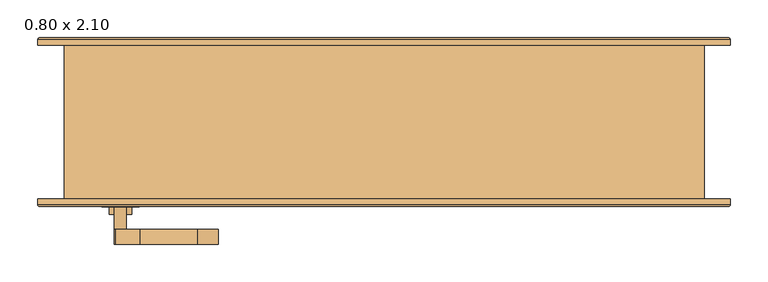
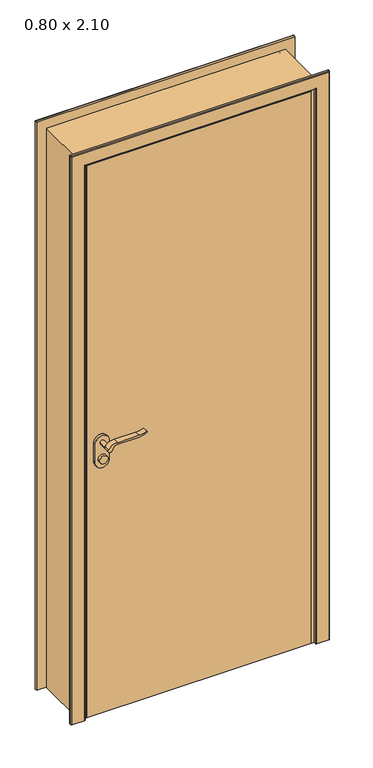
"""IFC4 building model written with IfcOpenShell, lengths in millimetres: door geometry, .CC_ND 300_PORTA SIMPLES DE ABRIR_COM EXTENSÃO : 0.80 x 2.10."""

from ifc_helpers import new_model, si_unit, point, frame, frame_2d, origin, origin_with_axes, place, context, project, spatial, polyline, circle_curve, ellipse_curve, trimmed, segment, composite_curve, outline, extrude, faceted_brep, source, transform, mapped, element, save
from ifc_brep_helpers import plane_surface, cylinder_surface, advanced_brep


def door_0_80_x_2_10_5db6a8b4(model_context):
    return source(origin(), model_context, "Body", "SolidModel", [
        extrude(outline(composite_curve([segment(trimmed(circle_curve(frame_2d((964.5, -350.0)), 15.0), [point((964.5, -335.0))], [point((964.5, -365.0))], False, "CARTESIAN"), True, "CONTINUOUS"), segment(trimmed(circle_curve(frame_2d((964.5, -350.0)), 15.0), [point((964.5, -365.0))], [point((964.5, -335.0))], False, "CARTESIAN"), True, "CONTINUOUS")], self_intersect=False)), frame((0.0, -137.9, 0.0), z_axis=(0.0, 1.0, 0.0), x_axis=(0.0, 0.0, 1.0)), (0.0, 0.0, 1.0), 10.0),
        extrude(outline(composite_curve([segment(trimmed(circle_curve(frame_2d((964.5, -350.0)), 15.0), [point((964.5, -335.0))], [point((964.5, -365.0))], False, "CARTESIAN"), True, "CONTINUOUS"), segment(trimmed(circle_curve(frame_2d((964.5, -350.0)), 15.0), [point((964.5, -365.0))], [point((964.5, -335.0))], False, "CARTESIAN"), True, "CONTINUOUS")], self_intersect=False)), frame((0.0, -77.9, 0.0), z_axis=(0.0, 1.0, 0.0), x_axis=(0.0, 0.0, 1.0)), (0.0, 0.0, 1.0), 10.0),
        extrude(outline(composite_curve([segment(trimmed(circle_curve(frame_2d((1024.5, -350.0)), 8.0), [point((1029.1523287, -356.5081363))], [point((1024.5, -342.0))], False, "CARTESIAN"), True, "CONTINUOUS"), segment(trimmed(circle_curve(frame_2d((1019.3738613, -324.6138099)), 18.1261387), [point((1024.5, -342.0))], [point((1037.5, -324.6138099))], True, "CARTESIAN"), True, "CONTINUOUS"), segment(polyline([(1037.5, -324.6138099), (1037.5, -248.3564091)]), True, "CONTINUOUS"), segment(trimmed(circle_curve(frame_2d((1096.7709207, -251.9396612)), 59.3791355), [point((1037.5, -248.3564091))], [point((1046.7135558, -220.0))], False, "CARTESIAN"), True, "CONTINUOUS"), segment(polyline([(1046.7135558, -220.0), (1049.5, -220.0)]), True, "CONTINUOUS"), segment(trimmed(circle_curve(frame_2d((1127.7850638, -248.4227909)), 83.2850902), [point((1049.5, -220.0))], [point((1044.5, -248.3564091))], True, "CARTESIAN"), True, "CONTINUOUS"), segment(polyline([(1044.5, -248.3564091), (1044.5, -324.6325667)]), True, "CONTINUOUS"), segment(trimmed(circle_curve(frame_2d((1007.2555521, -326.3324871)), 37.2832219), [point((1044.5, -324.6325667))], [point((1029.1523287, -356.5081363))], False, "CARTESIAN"), True, "CONTINUOUS")], self_intersect=False)), frame((0.0, -177.9, 0.0), z_axis=(0.0, 1.0, 0.0), x_axis=(0.0, 0.0, 1.0)), (0.0, 0.0, 1.0), 20.0),
        extrude(outline(composite_curve([segment(trimmed(circle_curve(frame_2d((1019.3738682, -324.6138122)), 18.1261318), [point((1024.4999903, -342.0))], [point((1037.5, -324.6138122))], True, "CARTESIAN"), True, "CONTINUOUS"), segment(polyline([(1037.5, -324.6138122), (1037.5, -248.3564091)]), True, "CONTINUOUS"), segment(trimmed(circle_curve(frame_2d((1096.7709207, -251.9396612)), 59.3791355), [point((1037.5, -248.3564091))], [point((1046.7135558, -220.0))], False, "CARTESIAN"), True, "CONTINUOUS"), segment(polyline([(1046.7135558, -220.0), (1049.5, -220.0)]), True, "CONTINUOUS"), segment(trimmed(circle_curve(frame_2d((1127.7850638, -248.4227909)), 83.2850902), [point((1049.5, -220.0))], [point((1044.5, -248.3564091))], True, "CARTESIAN"), True, "CONTINUOUS"), segment(polyline([(1044.5, -248.3564091), (1044.5, -324.6325667)]), True, "CONTINUOUS"), segment(trimmed(circle_curve(frame_2d((1007.2555521, -326.3324871)), 37.2832219), [point((1044.5, -324.6325667))], [point((1029.1523287, -356.5081363))], False, "CARTESIAN"), True, "CONTINUOUS"), segment(trimmed(circle_curve(frame_2d((1024.5, -350.0)), 8.0), [point((1029.1523287, -356.5081363))], [point((1024.4999903, -342.0))], False, "CARTESIAN"), True, "CONTINUOUS")], self_intersect=False)), frame((0.0, -47.9, 0.0), z_axis=(0.0, 1.0, 0.0), x_axis=(0.0, 0.0, 1.0)), (0.0, 0.0, 1.0), 20.0),
        extrude(outline(composite_curve([segment(trimmed(circle_curve(frame_2d((1024.5, -350.0)), 8.0), [point((1024.5, -342.0))], [point((1024.5, -358.0))], False, "CARTESIAN"), True, "CONTINUOUS"), segment(trimmed(circle_curve(frame_2d((1024.5, -350.0)), 8.0), [point((1024.5, -358.0))], [point((1024.5, -342.0))], False, "CARTESIAN"), True, "CONTINUOUS")], self_intersect=False)), frame((0.0, -157.9, 0.0), z_axis=(0.0, 1.0, 0.0), x_axis=(0.0, 0.0, 1.0)), (0.0, 0.0, 1.0), 30.0),
        extrude(outline(composite_curve([segment(trimmed(circle_curve(frame_2d((1024.5, -350.0)), 8.0), [point((1024.5, -342.0))], [point((1024.5, -358.0))], False, "CARTESIAN"), True, "CONTINUOUS"), segment(trimmed(circle_curve(frame_2d((1024.5, -350.0)), 8.0), [point((1024.5, -358.0))], [point((1024.5, -342.0))], False, "CARTESIAN"), True, "CONTINUOUS")], self_intersect=False)), frame((0.0, -77.9, 0.0), z_axis=(0.0, 1.0, 0.0), x_axis=(0.0, 0.0, 1.0)), (0.0, 0.0, 1.0), 30.0),
        extrude(outline(composite_curve([segment(trimmed(circle_curve(frame_2d((954.5, -350.0)), 25.0), [point((954.5, -375.0))], [point((954.5, -325.0))], False, "CARTESIAN"), True, "CONTINUOUS"), segment(polyline([(954.5, -325.0), (1024.5, -325.0)]), True, "CONTINUOUS"), segment(trimmed(circle_curve(frame_2d((1024.5, -350.0)), 25.0), [point((1024.5, -325.0))], [point((1024.5, -375.0))], False, "CARTESIAN"), True, "CONTINUOUS"), segment(polyline([(1024.5, -375.0), (954.5, -375.0)]), True, "CONTINUOUS")], self_intersect=False)), frame((0.0, -127.9, 0.0), z_axis=(0.0, 1.0, 0.0), x_axis=(0.0, 0.0, 1.0)), (0.0, 0.0, 1.0), 10.0),
        extrude(outline(composite_curve([segment(trimmed(circle_curve(frame_2d((954.5, -350.0)), 25.0), [point((954.5, -375.0))], [point((954.5, -325.0))], False, "CARTESIAN"), True, "CONTINUOUS"), segment(polyline([(954.5, -325.0), (1024.5, -325.0)]), True, "CONTINUOUS"), segment(trimmed(circle_curve(frame_2d((1024.5, -350.0)), 25.0), [point((1024.5, -325.0))], [point((1024.5, -375.0))], False, "CARTESIAN"), True, "CONTINUOUS"), segment(polyline([(1024.5, -375.0), (954.5, -375.0)]), True, "CONTINUOUS")], self_intersect=False)), frame((0.0, -87.9, 0.0), z_axis=(0.0, 1.0, 0.0), x_axis=(0.0, 0.0, 1.0)), (0.0, 0.0, 1.0), 10.0),
        faceted_brep([(392.0, 86.9, 0.0), (425.0, 86.9, 0.0), (425.0, -117.9, 0.0), (400.0, -117.9, 0.0), (400.0, -87.9, 0.0), (392.0, -87.9, 0.0), (392.0, 86.9, 2067.0), (-392.0, 86.9, 2067.0), (-392.0, 86.9, 0.0), (-425.0, 86.9, 0.0), (-425.0, 86.9, 2100.0), (425.0, 86.9, 2100.0), (425.0, -117.9, 2100.0), (-425.0, -117.9, 2100.0), (-425.0, -117.9, 0.0), (-400.0, -117.9, 0.0), (-400.0, -117.9, 2075.0), (400.0, -117.9, 2075.0), (400.0, -87.9, 2075.0), (-400.0, -87.9, 2075.0), (-400.0, -87.9, 0.0), (-392.0, -87.9, 0.0), (-392.0, -87.9, 2067.0), (392.0, -87.9, 2067.0)], [[[0, 1, 2, 3, 4, 5]], [[1, 0, 6, 7, 8, 9, 10, 11]], [[2, 1, 11, 12]], [[3, 2, 12, 13, 14, 15, 16, 17]], [[4, 3, 17, 18]], [[5, 4, 18, 19, 20, 21, 22, 23]], [[0, 5, 23, 6]], [[7, 22, 21, 8]], [[8, 21, 20, 15, 14, 9]], [[13, 10, 9, 14]], [[19, 16, 15, 20]], [[12, 11, 10, 13]], [[18, 17, 16, 19]], [[6, 23, 22, 7]]]),
        extrude(outline(polyline([(-400.0, -87.9), (400.0, -87.9), (400.0, -117.9), (-400.0, -117.9), (-400.0, -87.9)])), origin_with_axes(), (0.0, 0.0, 1.0), 2075.0),
        advanced_brep(
        [(-460.0, -117.9, 0.0), (-410.0, -117.9, 0.0), (-410.0, -124.9, 0.0), (-413.0, -127.9, 0.0), (-457.0, -127.9, 0.0), (-460.0, -124.9, 0.0), (-460.0, -117.9, 2135.0), (460.0, -117.9, 2135.0), (460.0, -117.9, 0.0), (410.0, -117.9, 0.0), (410.0, -117.9, 2085.0), (-410.0, -117.9, 2085.0), (-410.0, -124.9, 2085.0), (-413.0, -127.9, 2088.0), (413.0, -127.9, 2088.0), (413.0, -127.9, 0.0), (457.0, -127.9, 0.0), (457.0, -127.9, 2132.0), (-457.0, -127.9, 2132.0), (-460.0, -124.9, 2135.0), (460.0, -124.9, 2135.0), (460.0, -124.9, 0.0), (410.0, -124.9, 0.0), (410.0, -124.9, 2085.0)],
        [
            (0, 1),
            (1, 2),
            (2, 3, circle_curve(frame((-413.0, -124.9, 0.0), z_axis=(0.0, 0.0, -1.0), x_axis=(1.0, 0.0, 0.0)), 3.0)),
            (3, 4),
            (4, 5, circle_curve(frame((-457.0, -124.9, 0.0), z_axis=(0.0, 0.0, -1.0), x_axis=(1.0, 0.0, 0.0)), 3.0)),
            (5, 0),
            (0, 6),
            (6, 7),
            (7, 8),
            (8, 9),
            (9, 10),
            (10, 11),
            (11, 1),
            (11, 12),
            (12, 2),
            (12, 13, ellipse_curve(frame((-413.0, -124.9, 2088.0), z_axis=(-0.7071067811865475, 0.0, -0.7071067811865475), x_axis=(0.7071067811865474, 0.0, -0.7071067811865476)), 4.2426407, 3.0)),
            (13, 3),
            (13, 14),
            (14, 15),
            (15, 16),
            (16, 17),
            (17, 18),
            (18, 4),
            (18, 19, ellipse_curve(frame((-457.0, -124.9, 2132.0), z_axis=(-0.7071067811865475, 0.0, -0.7071067811865475), x_axis=(0.7071067811865474, 0.0, -0.7071067811865476)), 4.2426407, 3.0)),
            (19, 5),
            (19, 6),
            (7, 20),
            (20, 21),
            (21, 8),
            (21, 16, circle_curve(frame((457.0, -124.9, 0.0), z_axis=(0.0, 0.0, -1.0), x_axis=(-1.0, 0.0, 0.0)), 3.0)),
            (15, 22, circle_curve(frame((413.0, -124.9, 0.0), z_axis=(0.0, 0.0, -1.0), x_axis=(-1.0, 0.0, 0.0)), 3.0)),
            (22, 9),
            (23, 10),
            (22, 23),
            (14, 23, ellipse_curve(frame((413.0, -124.9, 2088.0), z_axis=(0.7071067811865475, 0.0, -0.7071067811865475), x_axis=(0.7071067811865474, 0.0, 0.7071067811865476)), 4.2426407, 3.0)),
            (20, 17, ellipse_curve(frame((457.0, -124.9, 2132.0), z_axis=(0.7071067811865475, 0.0, -0.7071067811865475), x_axis=(0.7071067811865474, 0.0, 0.7071067811865476)), 4.2426407, 3.0)),
            (23, 12),
            (19, 20),
        ],
        [
            plane_surface(frame((-410.0, -117.9, 0.0), z_axis=(0.0, 0.0, -1.0), x_axis=(0.0, 1.0, 0.0))),
            plane_surface(frame((-460.0, -117.9, 0.0), z_axis=(0.0, 1.0, 0.0), x_axis=(0.0, 0.0, 1.0))),
            plane_surface(frame((-410.0, -117.9, 0.0), z_axis=(1.0, 0.0, 0.0), x_axis=(0.0, 0.0, 1.0))),
            cylinder_surface(frame((-413.0, -124.9, 0.0), z_axis=(0.0, 0.0, -1.0), x_axis=(1.0, 0.0, 0.0)), 3.0),
            plane_surface(frame((-413.0, -127.9, 0.0), z_axis=(0.0, -1.0, 0.0), x_axis=(0.0, 0.0, 1.0))),
            cylinder_surface(frame((-457.0, -124.9, 0.0), z_axis=(0.0, 0.0, -1.0), x_axis=(1.0, 0.0, 0.0)), 3.0),
            plane_surface(frame((-460.0, -124.9, 0.0), z_axis=(-1.0, 0.0, 0.0), x_axis=(0.0, 0.0, 1.0))),
            plane_surface(frame((460.0, -124.9, 2135.0), z_axis=(1.0, 0.0, 0.0), x_axis=(0.0, 0.0, -1.0))),
            plane_surface(frame((410.0, -117.9, 0.0), z_axis=(0.0, 0.0, -1.0), x_axis=(0.0, 1.0, 0.0))),
            plane_surface(frame((410.0, -117.9, 2085.0), z_axis=(-1.0, 0.0, 0.0), x_axis=(0.0, 0.0, -1.0))),
            cylinder_surface(frame((413.0, -124.9, 2085.0), z_axis=(0.0, 0.0, 1.0), x_axis=(-1.0, 0.0, 0.0)), 3.0),
            cylinder_surface(frame((457.0, -124.9, 2085.0), z_axis=(0.0, 0.0, 1.0), x_axis=(-1.0, 0.0, 0.0)), 3.0),
            plane_surface(frame((-410.0, -117.9, 2085.0), z_axis=(0.0, 0.0, -1.0), x_axis=(1.0, 0.0, 0.0))),
            plane_surface(frame((-460.0, -124.9, 2135.0), z_axis=(0.0, 0.0, 1.0), x_axis=(1.0, 0.0, 0.0))),
            cylinder_surface(frame((-410.0, -124.9, 2088.0), z_axis=(-1.0, 0.0, 0.0), x_axis=(0.0, 0.0, -1.0)), 3.0),
            cylinder_surface(frame((-410.0, -124.9, 2132.0), z_axis=(-1.0, 0.0, 0.0), x_axis=(0.0, 0.0, -1.0)), 3.0),
        ],
        [
            (0, [[1, 2, 3, 4, 5, 6]]),
            (1, [[-1, 7, 8, 9, 10, 11, 12, 13]]),
            (2, [[-2, -13, 14, 15]]),
            (3, [[-3, -15, 16, 17]]),
            (4, [[-4, -17, 18, 19, 20, 21, 22, 23]]),
            (5, [[-5, -23, 24, 25]]),
            (6, [[-6, -25, 26, -7]]),
            (7, [[27, 28, 29, -9]]),
            (8, [[-29, 30, -20, 31, 32, -10]]),
            (9, [[33, -11, -32, 34]]),
            (10, [[35, -34, -31, -19]]),
            (11, [[36, -21, -30, -28]]),
            (12, [[-14, -12, -33, 37]]),
            (13, [[-26, 38, -27, -8]]),
            (14, [[-16, -37, -35, -18]]),
            (15, [[-24, -22, -36, -38]]),
        ],
    ),
        advanced_brep(
        [(460.0, 86.9, 0.0), (410.0, 86.9, 0.0), (410.0, 93.9157283, 0.0), (412.9842717, 96.9, 0.0), (457.0342217, 96.9, 0.0), (460.0, 93.9342217, 0.0), (460.0, 86.9, 2135.0), (-460.0, 86.9, 2135.0), (-460.0, 86.9, 0.0), (-410.0, 86.9, 0.0), (-410.0, 86.9, 2085.0), (410.0, 86.9, 2085.0), (410.0, 93.9157283, 2085.0), (412.9842717, 96.9, 2087.9842717), (-412.9842717, 96.9, 2087.9842717), (-412.9842717, 96.9, 0.0), (-457.0342217, 96.9, 0.0), (-457.0342217, 96.9, 2132.0342217), (457.0342217, 96.9, 2132.0342217), (460.0, 93.9342217, 2135.0), (-460.0, 93.9342217, 2135.0), (-460.0, 93.9342217, 0.0), (-410.0, 93.9157283, 0.0), (-410.0, 93.9157283, 2085.0)],
        [
            (0, 1),
            (1, 2),
            (2, 3, circle_curve(frame((412.9842717, 93.9157283, 0.0), z_axis=(0.0, 0.0, -1.0), x_axis=(1.0, 0.0, 0.0)), 2.9842717)),
            (3, 4),
            (4, 5, circle_curve(frame((457.0342217, 93.9342217, 0.0), z_axis=(0.0, 0.0, -1.0), x_axis=(1.0, 0.0, 0.0)), 2.9657783)),
            (5, 0),
            (0, 6),
            (6, 7),
            (7, 8),
            (8, 9),
            (9, 10),
            (10, 11),
            (11, 1),
            (11, 12),
            (12, 2),
            (12, 13, ellipse_curve(frame((412.9842717, 93.9157283, 2087.9842717), z_axis=(0.7071067811865475, 0.0, -0.7071067811865475), x_axis=(-0.7071067811865474, 0.0, -0.7071067811865476)), 4.2203975, 2.9842717)),
            (13, 3),
            (13, 14),
            (14, 15),
            (15, 16),
            (16, 17),
            (17, 18),
            (18, 4),
            (18, 19, ellipse_curve(frame((457.0342217, 93.9342217, 2132.0342217), z_axis=(0.7071067811865475, 0.0, -0.7071067811865475), x_axis=(-0.7071067811865474, 0.0, -0.7071067811865476)), 4.1942438, 2.9657783)),
            (19, 5),
            (19, 6),
            (7, 20),
            (20, 21),
            (21, 8),
            (21, 16, circle_curve(frame((-457.0342217, 93.9342217, 0.0), z_axis=(0.0, 0.0, -1.0), x_axis=(-1.0, 0.0, 0.0)), 2.9657783)),
            (15, 22, circle_curve(frame((-412.9842717, 93.9157283, 0.0), z_axis=(0.0, 0.0, -1.0), x_axis=(-1.0, 0.0, 0.0)), 2.9842717)),
            (22, 9),
            (23, 10),
            (22, 23),
            (14, 23, ellipse_curve(frame((-412.9842717, 93.9157283, 2087.9842717), z_axis=(-0.7071067811865475, 0.0, -0.7071067811865475), x_axis=(-0.7071067811865474, 0.0, 0.7071067811865476)), 4.2203975, 2.9842717)),
            (20, 17, ellipse_curve(frame((-457.0342217, 93.9342217, 2132.0342217), z_axis=(-0.7071067811865475, 0.0, -0.7071067811865475), x_axis=(-0.7071067811865474, 0.0, 0.7071067811865476)), 4.1942438, 2.9657783)),
            (23, 12),
            (19, 20),
        ],
        [
            plane_surface(frame((410.0, 86.9, 0.0), z_axis=(0.0, 0.0, -1.0), x_axis=(0.0, 1.0, 0.0))),
            plane_surface(frame((460.0, 86.9, 0.0), z_axis=(0.0, -1.0, 0.0), x_axis=(0.0, 0.0, 1.0))),
            plane_surface(frame((410.0, 86.9, 0.0), z_axis=(-1.0, 0.0, 0.0), x_axis=(0.0, 0.0, 1.0))),
            cylinder_surface(frame((412.9842717, 93.9157283, 0.0), z_axis=(0.0, 0.0, -1.0), x_axis=(1.0, 0.0, 0.0)), 2.9842717),
            plane_surface(frame((412.9842717, 96.9, 0.0), z_axis=(0.0, 1.0, 0.0), x_axis=(0.0, 0.0, 1.0))),
            cylinder_surface(frame((457.0342217, 93.9342217, 0.0), z_axis=(0.0, 0.0, -1.0), x_axis=(1.0, 0.0, 0.0)), 2.9657783),
            plane_surface(frame((460.0, 93.9342217, 0.0), z_axis=(1.0, 0.0, 0.0), x_axis=(0.0, 0.0, 1.0))),
            plane_surface(frame((-460.0, 93.9342217, 2135.0), z_axis=(-1.0, 0.0, 0.0), x_axis=(0.0, 0.0, -1.0))),
            plane_surface(frame((-410.0, 86.9, 0.0), z_axis=(0.0, 0.0, -1.0), x_axis=(0.0, 1.0, 0.0))),
            plane_surface(frame((-410.0, 86.9, 2085.0), z_axis=(1.0, 0.0, 0.0), x_axis=(0.0, 0.0, -1.0))),
            cylinder_surface(frame((-412.9842717, 93.9157283, 2085.0), z_axis=(0.0, 0.0, 1.0), x_axis=(-1.0, 0.0, 0.0)), 2.9842717),
            cylinder_surface(frame((-457.0342217, 93.9342217, 2085.0), z_axis=(0.0, 0.0, 1.0), x_axis=(-1.0, 0.0, 0.0)), 2.9657783),
            plane_surface(frame((410.0, 86.9, 2085.0), z_axis=(0.0, 0.0, -1.0), x_axis=(-1.0, 0.0, 0.0))),
            plane_surface(frame((460.0, 93.9342217, 2135.0), z_axis=(0.0, 0.0, 1.0), x_axis=(-1.0, 0.0, 0.0))),
            cylinder_surface(frame((410.0, 93.9157283, 2087.9842717), z_axis=(1.0, 0.0, 0.0), x_axis=(0.0, 0.0, 1.0)), 2.9842717),
            cylinder_surface(frame((410.0, 93.9342217, 2132.0342217), z_axis=(1.0, 0.0, 0.0), x_axis=(0.0, 0.0, 1.0)), 2.9657783),
        ],
        [
            (0, [[1, 2, 3, 4, 5, 6]]),
            (1, [[-1, 7, 8, 9, 10, 11, 12, 13]]),
            (2, [[-2, -13, 14, 15]]),
            (3, [[-3, -15, 16, 17]]),
            (4, [[-4, -17, 18, 19, 20, 21, 22, 23]]),
            (5, [[-5, -23, 24, 25]]),
            (6, [[-6, -25, 26, -7]]),
            (7, [[27, 28, 29, -9]]),
            (8, [[-29, 30, -20, 31, 32, -10]]),
            (9, [[33, -11, -32, 34]]),
            (10, [[35, -34, -31, -19]]),
            (11, [[36, -21, -30, -28]]),
            (12, [[-14, -12, -33, 37]]),
            (13, [[-26, 38, -27, -8]]),
            (14, [[-16, -37, -35, -18]]),
            (15, [[-24, -22, -36, -38]]),
        ],
    ),
    ])


if __name__ == "__main__":
    model = new_model("IFC4")
    model_context = context("Model", 3, world=origin())
    ifc_project = project(units=[si_unit("LENGTHUNIT", "METRE", prefix="MILLI")], contexts=[model_context])
    site = spatial("IfcSite", under=ifc_project)
    building = spatial("IfcBuilding", under=site)
    placement = place(None, origin())
    door_0_80_x_2_10_shape = door_0_80_x_2_10_5db6a8b4(model_context)
    element("IfcDoor", 1, ObjectType=".CC_ND 300_PORTA SIMPLES DE ABRIR_COM EXTENSÃO : 0.80 x 2.10", at=placement, inside=building, context=model_context, shape_type="MappedRepresentation", body=[
        mapped(door_0_80_x_2_10_shape, transform((0.0, 0.0, 0.0), x_axis=(1.0, 0.0, 0.0), y_axis=(0.0, 1.0, 0.0), z_axis=(0.0, 0.0, 1.0))),
    ])
    save(model, "model.ifc")

# Revit data of these elements
# Type ".CC_ND 300_PORTA SIMPLES DE ABRIR_COM EXTENSÃO : 0.80 x 2.10"
#   Type Mark = "153"
#   Analytic Construction = "<None>"
#   Rough Width = 0.85 m
#   Espessura moldura externa = 0.01 m
#   Espessura moldura interna = 0.01 m
#   Largura moldura = 0.05 m
#   Extensão acabamento exterior [instance default] = 0.00 m
#   Extensão acabamento interior [instance default] = 0.00 m
#   Espessura batente = 0.025 m
#   Thickness = 0.03 m
#   Altura batente = 2.085 m
#   Aux Arco [instance default] = 0.80 m
#   Rough Height = 2.125 m
#   Height = 2.10 m
#   Width = 0.80 m
#   Moldura interna [instance default] = yes
#   Moldura externa [instance default] = yes
#   Porta = .MADEIRA COM PINTURA ESMALTE BRANCO ACETINADO
#   Moldura = .MADEIRA COM PINTURA ESMALTE BRANCO ACETINADO
#   Maçaneta = .ALUMÍNIO
#   Batente = .MADEIRA COM PINTURA ESMALTE BRANCO ACETINADO
#   Function = (empty or 0)
#   Wall Closure = (empty or 0)
# Element 1 (IfcDoor, ".CC_ND 300_PORTA SIMPLES DE ABRIR_COM EXTENSÃO : 0.80 x 2.10")
#   Extensão acabamento interior = 0.031 m
#   Aux Arco = 0.831 m
#   Materials on its faces: ".MADEIRA COM PINTURA ESMALTE BRANCO ACETINADO", ".ALUMÍNIO"
# Materials
#   ".MADEIRA COM PINTURA ESMALTE BRANCO ACETINADO": class ".CC_MADEIRAS", colour RGB 240 240 240, transparency 0, Description = "Madeira com pintura esmalte branco acetinado.", Cost = 0
#   ".ALUMÍNIO": class "CC_METAIS", colour RGB 244 244 244, transparency 0, Description = "Material alumínio", Cost = 0
